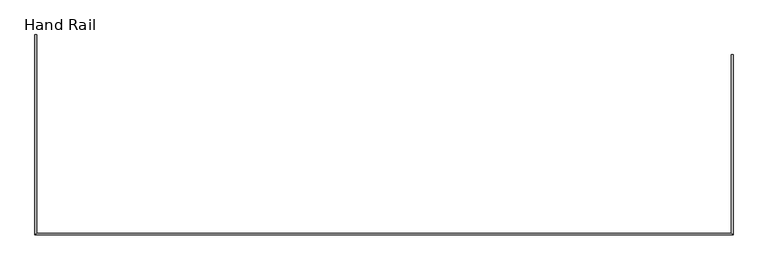
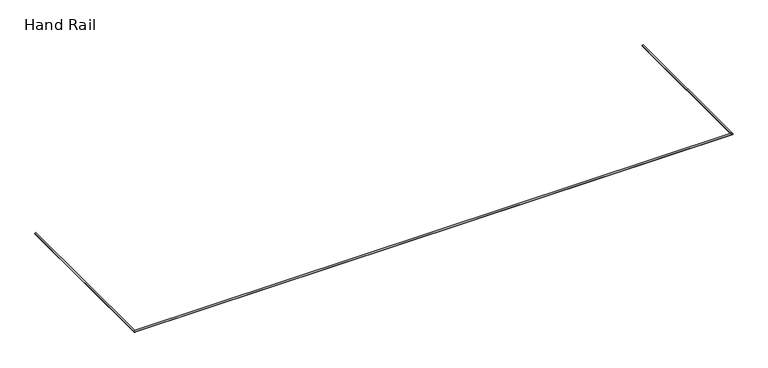
"""IFC4 building model written with IfcOpenShell, lengths in millimetres: railing geometry, Hand Rail."""

from ifc_helpers import new_model, si_unit, frame, origin, place, context, project, spatial, circle_curve, ellipse_curve, source, transform, mapped, element, save
from ifc_brep_helpers import plane_surface, cylinder_surface, advanced_brep


def hand_rail_ea9dd5f3(model_context):
    return source(origin(), model_context, "Body", "AdvancedBrep", [
        advanced_brep(
        [(-10864.834448, 67.4947073, 4521.5181462), (-10890.234448, 67.4947073, 4521.5181462), (-10864.834448, -2966.4271465, 4521.5181462), (-10890.234448, -2991.8271465, 4521.5181462), (-265.3743061, -2966.4271465, 4521.5181462), (-239.9743061, -2991.8271465, 4521.5181462), (-265.3743061, -237.3052927, 4521.5181462), (-239.9743061, -237.3052927, 4521.5181462)],
        [
            (0, 1, circle_curve(frame((-10877.534448, 67.4947073, 4521.5181462), z_axis=(0.0, 1.0, 0.0), x_axis=(-1.0, 0.0, 0.0)), 12.7)),
            (1, 0, circle_curve(frame((-10877.534448, 67.4947073, 4521.5181462), z_axis=(0.0, 1.0, 0.0), x_axis=(-1.0, 0.0, 0.0)), 12.7)),
            (0, 2),
            (2, 3, ellipse_curve(frame((-10877.534448, -2979.1271465, 4521.5181462), z_axis=(-0.7071067811865475, 0.7071067811865475, 0.0), x_axis=(0.7071067811865474, 0.7071067811865476, 0.0)), 17.9605122, 12.7)),
            (3, 1),
            (3, 2, ellipse_curve(frame((-10877.534448, -2979.1271465, 4521.5181462), z_axis=(-0.7071067811865475, 0.7071067811865475, 0.0), x_axis=(0.7071067811865474, 0.7071067811865476, 0.0)), 17.9605122, 12.7)),
            (2, 4),
            (4, 5, ellipse_curve(frame((-252.6743061, -2979.1271465, 4521.5181462), z_axis=(-0.7071067811865475, -0.7071067811865476, 0.0), x_axis=(-0.7071067811865476, 0.7071067811865475, 0.0)), 17.9605122, 12.7)),
            (5, 3),
            (5, 4, ellipse_curve(frame((-252.6743061, -2979.1271465, 4521.5181462), z_axis=(-0.7071067811865475, -0.7071067811865476, 0.0), x_axis=(-0.7071067811865476, 0.7071067811865475, 0.0)), 17.9605122, 12.7)),
            (6, 7, circle_curve(frame((-252.6743061, -237.3052927, 4521.5181462), z_axis=(0.0, 1.0, 0.0), x_axis=(1.0, 0.0, 0.0)), 12.7)),
            (7, 6, circle_curve(frame((-252.6743061, -237.3052927, 4521.5181462), z_axis=(0.0, 1.0, 0.0), x_axis=(1.0, 0.0, 0.0)), 12.7)),
            (4, 6),
            (7, 5),
        ],
        [
            plane_surface(frame((-10877.534448, 67.4947073, 4534.2181462), z_axis=(0.0, 1.0, 0.0), x_axis=(0.0, 0.0, -1.0))),
            cylinder_surface(frame((-10877.534448, 67.4947073, 4521.5181462), z_axis=(0.0, 1.0, 0.0), x_axis=(-1.0, 0.0, 0.0)), 12.7),
            cylinder_surface(frame((-10877.534448, -2979.1271465, 4521.5181462), z_axis=(-1.0, 0.0, 0.0), x_axis=(0.0, -1.0, 0.0)), 12.7),
            plane_surface(frame((-252.6743061, -237.3052927, 4534.2181462), z_axis=(0.0, 1.0, 0.0), x_axis=(0.0, 0.0, 1.0))),
            cylinder_surface(frame((-252.6743061, -2979.1271465, 4521.5181462), z_axis=(0.0, -1.0, 0.0), x_axis=(1.0, 0.0, 0.0)), 12.7),
        ],
        [
            (0, [[1, 2]]),
            (1, [[-1, 3, 4, 5]]),
            (1, [[-2, -5, 6, -3]]),
            (2, [[-4, 7, 8, 9]]),
            (2, [[-6, -9, 10, -7]]),
            (3, [[11, 12]]),
            (4, [[-8, 13, -12, 14]]),
            (4, [[-10, -14, -11, -13]]),
        ],
    ),
    ])


if __name__ == "__main__":
    model = new_model("IFC4")
    model_context = context("Model", 3, world=origin())
    ifc_project = project(units=[si_unit("LENGTHUNIT", "METRE", prefix="MILLI")], contexts=[model_context])
    site = spatial("IfcSite", under=ifc_project)
    building = spatial("IfcBuilding", under=site)
    placement = place(None, origin())
    hand_rail_shape = hand_rail_ea9dd5f3(model_context)
    element("IfcRailing", 1, ObjectType="Hand Rail", at=placement, inside=building, context=model_context, shape_type="MappedRepresentation", body=[
        mapped(hand_rail_shape, transform((0.0, 0.0, 0.0), x_axis=(1.0, 0.0, 0.0), y_axis=(0.0, 1.0, 0.0), z_axis=(0.0, 0.0, 1.0))),
    ])
    save(model, "model.ifc")

# Revit data of these elements
# Element 1 (IfcRailing, "Hand Rail")
#   Materials on its faces: "RAILING STEEL"
# Materials
#   "RAILING STEEL": class "Metal", colour RGB 16 16 15, transparency 0, Description = "Structural steel, ASTM A36 Grade B, mill finish", Cost = 0
